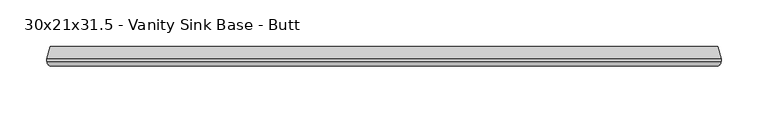
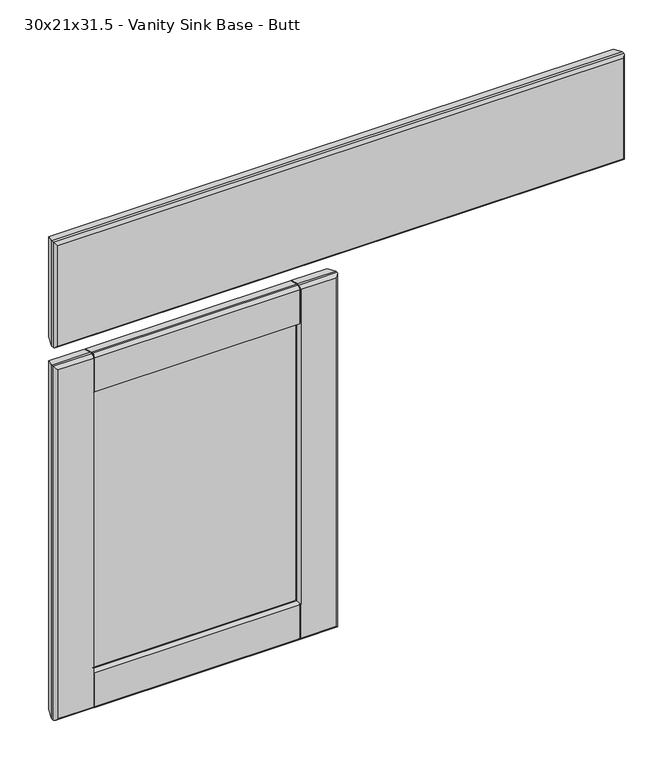
"""IFC4 building model written with IfcOpenShell, lengths in millimetres: furniture geometry, Cabinet-Base-Merillat-Double_Door-Marlin : 30x21x31.5 - Vanity Sink Base - Butt."""

from ifc_helpers import new_model, si_unit, frame, origin, place, context, project, spatial, polyline, circle_curve, ellipse_curve, outline, extrude, source, transform, mapped, element, save
from ifc_brep_helpers import plane_surface, cylinder_surface, advanced_brep


def furniture_30x21x31_5_vanity_sink_base_butt_a027e388(model_context):
    return source(origin(), model_context, "Body", "SolidModel", [
        advanced_brep(
        [(-336.9408026, -629.92, 771.6035075), (-336.9408026, -629.92, 638.0964925), (374.4162124, -629.92, 638.0964925), (374.4162124, -629.92, 771.6035075), (-336.5320951, -609.6, 638.5052), (-336.5320951, -609.6, 771.1948), (374.0075049, -609.6, 771.1948), (374.0075049, -609.6, 638.5052), (-340.0372951, -625.4496, 774.7), (-340.0372951, -622.681, 774.7), (-340.0372951, -622.681, 635.0), (-340.0372951, -625.4496, 635.0), (377.5127049, -622.681, 635.0), (377.5127049, -625.4496, 635.0), (377.5127049, -622.681, 774.7), (377.5127049, -625.4496, 774.7)],
        [
            (0, 1),
            (1, 2),
            (2, 3),
            (3, 0),
            (4, 5),
            (5, 6),
            (6, 7),
            (7, 4),
            (8, 9),
            (9, 10),
            (10, 11),
            (11, 8),
            (10, 12),
            (12, 13),
            (13, 11),
            (12, 14),
            (14, 15),
            (15, 13),
            (8, 15),
            (14, 9),
            (11, 1, ellipse_curve(frame((-335.2620951, -625.4496, 639.7752), z_axis=(-0.7071067811865475, 0.0, 0.7071067811865475), x_axis=(-0.7071067811865474, 0.0, -0.7071067811865476)), 6.7531526, 4.7752)),
            (0, 8, ellipse_curve(frame((-335.2620951, -625.4496, 769.9248), z_axis=(-0.7071067811865475, 0.0, -0.7071067811865475), x_axis=(0.7071067811865474, 0.0, -0.7071067811865476)), 6.7531526, 4.7752)),
            (4, 10),
            (9, 5),
            (13, 2, ellipse_curve(frame((372.7375049, -625.4496, 639.7752), z_axis=(-0.7071067811865475, 0.0, -0.7071067811865475), x_axis=(0.7071067811865476, 0.0, -0.7071067811865474)), 6.7531526, 4.7752)),
            (7, 12),
            (15, 3, ellipse_curve(frame((372.7375049, -625.4496, 769.9248), z_axis=(0.7071067811865475, 0.0, -0.7071067811865475), x_axis=(0.7071067811865474, 0.0, 0.7071067811865476)), 6.7531526, 4.7752)),
            (6, 14),
        ],
        [
            plane_surface(frame((-340.0372951, -629.92, 774.7), z_axis=(0.0, -1.0, 0.0), x_axis=(0.0, 0.0, -1.0))),
            plane_surface(frame((-340.0372951, -609.6, 774.7), z_axis=(0.0, 1.0, 0.0), x_axis=(0.0, 0.0, 1.0))),
            plane_surface(frame((-340.0372951, -629.92, 774.7), z_axis=(-1.0, 0.0, 0.0), x_axis=(0.0, 1.0, 0.0))),
            plane_surface(frame((-340.0372951, -629.92, 635.0), z_axis=(0.0, 0.0, -1.0), x_axis=(0.0, 1.0, 0.0))),
            plane_surface(frame((377.5127049, -629.92, 635.0), z_axis=(1.0, 0.0, 0.0), x_axis=(0.0, 1.0, 0.0))),
            plane_surface(frame((377.5127049, -629.92, 774.7), z_axis=(0.0, 0.0, 1.0), x_axis=(0.0, 1.0, 0.0))),
            cylinder_surface(frame((-335.2620951, -625.4496, 774.7), z_axis=(0.0, 0.0, -1.0), x_axis=(0.0, 1.0, 0.0)), 4.7752),
            plane_surface(frame((-340.0372951, -622.681, 774.7), z_axis=(-0.9659229350723619, 0.25882983502910506, 0.0), x_axis=(0.0, 0.0, -1.0))),
            cylinder_surface(frame((-340.0372951, -625.4496, 639.7752), z_axis=(1.0, 0.0, 0.0), x_axis=(0.0, 1.0, 0.0)), 4.7752),
            plane_surface(frame((-340.0372951, -622.681, 635.0), z_axis=(0.0, 0.25882983502910506, -0.9659229350723619), x_axis=(1.0, 0.0, 0.0))),
            cylinder_surface(frame((372.7375049, -625.4496, 635.0), z_axis=(0.0, 0.0, 1.0), x_axis=(0.0, 1.0, 0.0)), 4.7752),
            plane_surface(frame((377.5127049, -622.681, 635.0), z_axis=(0.9659229350723619, 0.25882983502910506, 0.0), x_axis=(0.0, 0.0, 1.0))),
            cylinder_surface(frame((377.5127049, -625.4496, 769.9248), z_axis=(-1.0, 0.0, 0.0), x_axis=(0.0, 1.0, 0.0)), 4.7752),
            plane_surface(frame((377.5127049, -622.681, 774.7), z_axis=(0.0, 0.25882983502910506, 0.9659229350723619), x_axis=(-1.0, 0.0, 0.0))),
        ],
        [
            (0, [[1, 2, 3, 4]]),
            (1, [[5, 6, 7, 8]]),
            (2, [[9, 10, 11, 12]]),
            (3, [[-11, 13, 14, 15]]),
            (4, [[-14, 16, 17, 18]]),
            (5, [[-9, 19, -17, 20]]),
            (6, [[21, -1, 22, -12]]),
            (7, [[23, -10, 24, -5]]),
            (8, [[-21, -15, 25, -2]]),
            (9, [[-23, -8, 26, -13]]),
            (10, [[-25, -18, 27, -3]]),
            (11, [[-26, -7, 28, -16]]),
            (12, [[-22, -4, -27, -19]]),
            (13, [[-24, -20, -28, -6]]),
        ],
    ),
        advanced_brep(
        [(-340.0372951, -625.4496, 609.6), (-340.0372951, -625.4496, 139.7), (-336.9408026, -629.92, 142.7964925), (-336.9408026, -629.92, 606.5035075), (-340.0372951, -622.681, 609.6), (-340.0372951, -622.681, 139.7), (-336.5320951, -609.6, 606.0948), (-336.5320951, -609.6, 143.2052), (-291.8361323, -609.6, 561.3988372), (-291.4660006, -610.39375, 561.0287055), (-289.3848416, -614.85681, 558.9475465), (-289.3848416, -614.85681, 190.3524535), (-291.4660006, -610.39375, 188.2712945), (-291.8361323, -609.6, 187.9011628), (-290.784611, -617.0969093, 560.347316), (-290.784611, -617.0969093, 188.952684), (-305.1122951, -617.347, 574.675), (-305.1122951, -617.347, 174.625), (-305.1122951, -622.173, 574.675), (-305.1122951, -622.173, 174.625), (-290.784611, -622.4230907, 560.347316), (-290.784611, -622.4230907, 188.952684), (-289.3848416, -624.66319, 558.9475465), (-289.3848416, -624.66319, 190.3524535), (-291.4660006, -629.12625, 561.0287055), (-291.8332649, -629.9138508, 561.3959698), (-291.8361323, -629.92, 187.9011628), (-291.4660006, -629.12625, 188.2712945), (14.0537124, -629.92, 142.7964925), (-31.0140137, -629.92, 142.7964925), (-31.0140137, -625.4496, 139.7), (17.1502049, -625.4496, 139.7), (-291.8332649, -625.4496, 139.7), (-291.8332649, -629.92, 142.7964925), (-290.2457649, -625.4496, 139.7), (-32.6015137, -625.4496, 139.7), (-32.6015137, -629.92, 142.7964925), (-290.2457649, -629.92, 142.7964925), (-31.0140137, -622.681, 139.7), (17.1502049, -622.681, 139.7), (-291.8332649, -622.681, 139.7), (-290.2457649, -622.681, 139.7), (-32.6015137, -622.681, 139.7), (-31.0140137, -609.6, 143.2052), (13.6450049, -609.6, 143.2052), (-290.2457649, -609.6, 143.2052), (-32.6015137, -609.6, 143.2052), (-291.8332649, -609.6, 143.2052), (-33.5022486, -614.85681, 190.3524535), (-31.4210895, -610.39375, 188.2712945), (-32.6015137, -610.39375, 188.2712945), (-32.6015137, -609.6, 187.9011628), (-290.2457649, -609.6, 187.9011628), (-290.2457649, -610.39375, 188.2712945), (-32.1024791, -617.0969093, 188.952684), (-17.7747951, -617.347, 174.625), (-17.7747951, -622.173, 174.625), (-32.1024791, -622.4230907, 188.952684), (-33.5022486, -624.66319, 190.3524535), (-290.2457649, -629.12625, 188.2712945), (-290.2457649, -629.92, 187.9011628), (-32.6015137, -629.92, 187.9011628), (-32.6015137, -629.12625, 188.2712945), (-31.4210895, -629.12625, 188.2712945), (17.1502049, -625.4496, 609.6), (14.0537124, -629.92, 606.5035075), (17.1502049, -622.681, 609.6), (13.6450049, -609.6, 606.0948), (-31.0509578, -609.6, 187.9011628), (-33.5022486, -614.85681, 558.9475465), (-31.4210895, -610.39375, 561.0287055), (-31.0509578, -609.6, 561.3988372), (-32.1024791, -617.0969093, 560.347316), (-17.7747951, -617.347, 574.675), (-17.7747951, -622.173, 574.675), (-32.1024791, -622.4230907, 560.347316), (-33.5022486, -624.66319, 558.9475465), (-31.0509578, -629.92, 187.9011628), (-31.0509578, -629.92, 561.3988372), (-31.4210895, -629.12625, 561.0287055), (-291.8332649, -629.92, 606.5035075), (-291.8332649, -625.4496, 609.6), (-31.0140137, -625.4496, 609.6), (-31.0140137, -629.92, 606.5035075), (-32.6015137, -625.4496, 609.6), (-290.2457649, -625.4496, 609.6), (-290.2457649, -629.92, 606.5035075), (-32.6015137, -629.92, 606.5035075), (-291.8332649, -622.681, 609.6), (-31.0140137, -622.681, 609.6), (-32.6015137, -622.681, 609.6), (-290.2457649, -622.681, 609.6), (-291.8332649, -609.6, 606.0948), (-31.0140137, -609.6, 606.0948), (-32.6015137, -609.6, 606.0948), (-290.2457649, -609.6, 606.0948), (-32.6015137, -609.6, 561.3988372), (-290.2457649, -609.6, 561.3988372), (-290.2457649, -610.39375, 561.0287055), (-32.6015137, -610.39375, 561.0287055), (-32.6015137, -629.12625, 561.0287055), (-32.6015137, -629.92, 561.3988372), (-290.2457649, -629.92, 561.3988372), (-290.2457649, -629.12625, 561.0287055), (-32.6015137, -629.12625, 606.3526052), (-32.6015137, -625.4496, 608.80625), (-32.6015137, -622.7855037, 608.80625), (-32.6015137, -610.39375, 605.4857412), (-31.0140137, -610.39375, 561.0287055), (-31.0140137, -610.39375, 605.4857412), (-31.0140137, -622.7855037, 608.80625), (-31.0140137, -625.4496, 608.80625), (-31.0140137, -629.12625, 606.3526052), (-31.0140137, -629.12625, 561.0287055), (-291.8332649, -629.12625, 561.0287055), (-291.8332649, -629.12625, 606.3526052), (-291.8332649, -625.4496, 608.80625), (-291.8332649, -622.7855037, 608.80625), (-291.8332649, -610.39375, 605.4857412), (-291.8332649, -610.39375, 561.0287055), (-290.2457649, -610.39375, 605.4857412), (-290.2457649, -622.7855037, 608.80625), (-290.2457649, -625.4496, 608.80625), (-290.2457649, -629.12625, 606.3526052), (-291.8332649, -610.39375, 188.2712945), (-291.8332649, -610.39375, 143.8142588), (-291.8332649, -622.7855037, 140.49375), (-291.8332649, -625.4496, 140.49375), (-291.8332649, -629.12625, 142.9473948), (-291.8332649, -629.12625, 188.2712945), (-290.2457649, -629.12625, 142.9473948), (-290.2457649, -625.4496, 140.49375), (-290.2457649, -622.7855037, 140.49375), (-290.2457649, -610.39375, 143.8142588), (-32.6015137, -610.39375, 143.8142588), (-32.6015137, -622.7855037, 140.49375), (-32.6015137, -625.4496, 140.49375), (-32.6015137, -629.12625, 142.9473948), (-31.0140137, -629.12625, 188.2712945), (-31.0140137, -629.12625, 142.9473948), (-31.0140137, -625.4496, 140.49375), (-31.0140137, -622.7855037, 140.49375), (-31.0140137, -610.39375, 143.8142588), (-31.0140137, -610.39375, 188.2712945)],
        [
            (0, 1),
            (1, 2, ellipse_curve(frame((-335.2620951, -625.4496, 144.4752), z_axis=(-0.7071067811865475, 0.0, 0.7071067811865475), x_axis=(0.7071067811865474, 0.0, 0.7071067811865476)), 6.7531526, 4.7752)),
            (2, 3),
            (3, 0, ellipse_curve(frame((-335.2620951, -625.4496, 604.8248), z_axis=(-0.7071067811865475, 0.0, -0.7071067811865475), x_axis=(-0.7071067811865474, 0.0, 0.7071067811865476)), 6.7531526, 4.7752)),
            (0, 4),
            (4, 5),
            (5, 1),
            (4, 6),
            (6, 7),
            (7, 5),
            (8, 9),
            (9, 10),
            (10, 11),
            (11, 12),
            (12, 13),
            (13, 8),
            (10, 14, ellipse_curve(frame((-290.8120951, -615.5223492, 560.3748), z_axis=(-0.7071067811865475, 0.0, -0.7071067811865475), x_axis=(-0.7071067811865474, 0.0, 0.7071067811865476)), 2.2271035, 1.5748)),
            (14, 15),
            (15, 11, ellipse_curve(frame((-290.8120951, -615.5223492, 188.9252), z_axis=(-0.7071067811865475, 0.0, 0.7071067811865475), x_axis=(0.7071067811865474, 0.0, 0.7071067811865476)), 2.2271035, 1.5748)),
            (14, 16),
            (16, 17),
            (17, 15),
            (16, 18),
            (18, 19),
            (19, 17),
            (18, 20),
            (20, 21),
            (21, 19),
            (20, 22, ellipse_curve(frame((-290.8120951, -623.9976508, 560.3748), z_axis=(-0.7071067811865475, 0.0, -0.7071067811865475), x_axis=(-0.7071067811865474, 0.0, 0.7071067811865476)), 2.2271035, 1.5748)),
            (22, 23),
            (23, 21, ellipse_curve(frame((-290.8120951, -623.9976508, 188.9252), z_axis=(-0.7071067811865475, 0.0, 0.7071067811865475), x_axis=(0.7071067811865474, 0.0, 0.7071067811865476)), 2.2271035, 1.5748)),
            (22, 24),
            (24, 25),
            (25, 26),
            (26, 27),
            (27, 23),
            (28, 29),
            (29, 30, circle_curve(frame((-31.0140137, -625.4496, 144.4752), z_axis=(1.0, 0.0, 0.0), x_axis=(0.0, 1.0, 0.0)), 4.7752)),
            (30, 31),
            (31, 28, ellipse_curve(frame((12.3750049, -625.4496, 144.4752), z_axis=(-0.7071067811865475, 0.0, -0.7071067811865475), x_axis=(-0.7071067811865476, 0.0, 0.7071067811865474)), 6.7531526, 4.7752)),
            (1, 32),
            (32, 33, circle_curve(frame((-291.8332649, -625.4496, 144.4752), z_axis=(-1.0, 0.0, 0.0), x_axis=(0.0, 1.0, 0.0)), 4.7752)),
            (33, 2),
            (34, 35),
            (35, 36, circle_curve(frame((-32.6015137, -625.4496, 144.4752), z_axis=(-1.0, 0.0, 0.0), x_axis=(0.0, 1.0, 0.0)), 4.7752)),
            (36, 37),
            (37, 34, circle_curve(frame((-290.2457649, -625.4496, 144.4752), z_axis=(1.0, 0.0, 0.0), x_axis=(0.0, 1.0, 0.0)), 4.7752)),
            (30, 38),
            (38, 39),
            (39, 31),
            (5, 40),
            (40, 32),
            (41, 42),
            (42, 35),
            (34, 41),
            (38, 43),
            (43, 44),
            (44, 39),
            (45, 46),
            (46, 42),
            (41, 45),
            (7, 47),
            (47, 40),
            (48, 49),
            (49, 50),
            (50, 51),
            (51, 52),
            (52, 53),
            (53, 12),
            (11, 48),
            (15, 54),
            (54, 48, ellipse_curve(frame((-32.0749951, -615.5223492, 188.9252), z_axis=(-0.7071067811865475, 0.0, -0.7071067811865475), x_axis=(-0.7071067811865476, 0.0, 0.7071067811865474)), 2.2271035, 1.5748)),
            (17, 55),
            (55, 54),
            (19, 56),
            (56, 55),
            (21, 57),
            (57, 56),
            (23, 58),
            (58, 57, ellipse_curve(frame((-32.0749951, -623.9976508, 188.9252), z_axis=(-0.7071067811865475, 0.0, -0.7071067811865475), x_axis=(-0.7071067811865476, 0.0, 0.7071067811865474)), 2.2271035, 1.5748)),
            (27, 59),
            (59, 60),
            (60, 61),
            (61, 62),
            (62, 63),
            (63, 58),
            (31, 64),
            (64, 65, ellipse_curve(frame((12.3750049, -625.4496, 604.8248), z_axis=(0.7071067811865475, 0.0, -0.7071067811865475), x_axis=(-0.7071067811865474, 0.0, -0.7071067811865476)), 6.7531526, 4.7752)),
            (65, 28),
            (39, 66),
            (66, 64),
            (44, 67),
            (67, 66),
            (68, 49),
            (48, 69),
            (69, 70),
            (70, 71),
            (71, 68),
            (54, 72),
            (72, 69, ellipse_curve(frame((-32.0749951, -615.5223492, 560.3748), z_axis=(0.7071067811865475, 0.0, -0.7071067811865475), x_axis=(-0.7071067811865474, 0.0, -0.7071067811865476)), 2.2271035, 1.5748)),
            (55, 73),
            (73, 72),
            (56, 74),
            (74, 73),
            (57, 75),
            (75, 74),
            (58, 76),
            (76, 75, ellipse_curve(frame((-32.0749951, -623.9976508, 560.3748), z_axis=(0.7071067811865475, 0.0, -0.7071067811865475), x_axis=(-0.7071067811865474, 0.0, -0.7071067811865476)), 2.2271035, 1.5748)),
            (63, 77),
            (77, 78),
            (78, 79),
            (79, 76),
            (3, 80),
            (80, 81, circle_curve(frame((-291.8332649, -625.4496, 604.8248), z_axis=(-1.0, 0.0, 0.0), x_axis=(0.0, 1.0, 0.0)), 4.7752)),
            (81, 0),
            (64, 82),
            (82, 83, circle_curve(frame((-31.0140137, -625.4496, 604.8248), z_axis=(1.0, 0.0, 0.0), x_axis=(0.0, 1.0, 0.0)), 4.7752)),
            (83, 65),
            (84, 85),
            (85, 86, circle_curve(frame((-290.2457649, -625.4496, 604.8248), z_axis=(1.0, 0.0, 0.0), x_axis=(0.0, 1.0, 0.0)), 4.7752)),
            (86, 87),
            (87, 84, circle_curve(frame((-32.6015137, -625.4496, 604.8248), z_axis=(-1.0, 0.0, 0.0), x_axis=(0.0, 1.0, 0.0)), 4.7752)),
            (81, 88),
            (88, 4),
            (66, 89),
            (89, 82),
            (90, 91),
            (91, 85),
            (84, 90),
            (88, 92),
            (92, 6),
            (67, 93),
            (93, 89),
            (94, 95),
            (95, 91),
            (90, 94),
            (51, 46),
            (45, 52),
            (43, 68),
            (71, 93),
            (92, 8),
            (13, 47),
            (96, 97),
            (97, 95),
            (94, 96),
            (9, 98),
            (98, 97),
            (96, 99),
            (99, 70),
            (69, 10),
            (72, 14),
            (73, 16),
            (74, 18),
            (75, 20),
            (76, 22),
            (79, 100),
            (100, 101),
            (101, 102),
            (102, 103),
            (103, 24),
            (33, 26),
            (25, 80),
            (36, 61),
            (60, 37),
            (83, 78),
            (77, 29),
            (86, 102),
            (101, 87),
            (100, 104),
            (104, 105, circle_curve(frame((-32.6015137, -625.4496, 604.8248), z_axis=(-1.0, 0.0, 0.0), x_axis=(0.0, 0.0, 1.0)), 3.98145)),
            (105, 106),
            (106, 107),
            (107, 99),
            (71, 108),
            (108, 109),
            (109, 110),
            (110, 111),
            (111, 112, circle_curve(frame((-31.0140137, -625.4496, 604.8248), z_axis=(1.0, 0.0, 0.0), x_axis=(0.0, 0.0, 1.0)), 3.98145)),
            (112, 113),
            (113, 78),
            (113, 79),
            (112, 104),
            (111, 105),
            (110, 106),
            (109, 107),
            (108, 70),
            (25, 114),
            (114, 115),
            (115, 116, circle_curve(frame((-291.8332649, -625.4496, 604.8248), z_axis=(-1.0, 0.0, 0.0), x_axis=(0.0, 0.0, 1.0)), 3.98145)),
            (116, 117),
            (117, 118),
            (118, 119),
            (119, 8),
            (98, 120),
            (120, 121),
            (121, 122),
            (122, 123, circle_curve(frame((-290.2457649, -625.4496, 604.8248), z_axis=(1.0, 0.0, 0.0), x_axis=(0.0, 0.0, 1.0)), 3.98145)),
            (123, 103),
            (24, 114),
            (123, 115),
            (122, 116),
            (121, 117),
            (120, 118),
            (9, 119),
            (13, 124),
            (124, 125),
            (125, 126),
            (126, 127),
            (127, 128, circle_curve(frame((-291.8332649, -625.4496, 144.4752), z_axis=(-1.0, 0.0, 0.0), x_axis=(0.0, 0.0, 1.0)), 3.98145)),
            (128, 129),
            (129, 26),
            (59, 130),
            (130, 131, circle_curve(frame((-290.2457649, -625.4496, 144.4752), z_axis=(1.0, 0.0, 0.0), x_axis=(0.0, 0.0, 1.0)), 3.98145)),
            (131, 132),
            (132, 133),
            (133, 53),
            (12, 124),
            (133, 125),
            (132, 126),
            (131, 127),
            (130, 128),
            (27, 129),
            (50, 134),
            (134, 135),
            (135, 136),
            (136, 137, circle_curve(frame((-32.6015137, -625.4496, 144.4752), z_axis=(-1.0, 0.0, 0.0), x_axis=(0.0, 0.0, 1.0)), 3.98145)),
            (137, 62),
            (138, 139),
            (139, 140, circle_curve(frame((-31.0140137, -625.4496, 144.4752), z_axis=(1.0, 0.0, 0.0), x_axis=(0.0, 0.0, 1.0)), 3.98145)),
            (140, 141),
            (141, 142),
            (142, 143),
            (143, 68),
            (77, 138),
            (63, 138),
            (143, 49),
            (142, 134),
            (141, 135),
            (140, 136),
            (139, 137),
        ],
        [
            cylinder_surface(frame((-335.2620951, -625.4496, 609.6), z_axis=(0.0, 0.0, 1.0), x_axis=(0.0, 1.0, 0.0)), 4.7752),
            plane_surface(frame((-340.0372951, -625.4496, 609.6), z_axis=(-1.0, 0.0, 0.0), x_axis=(0.0, 0.0, -1.0))),
            plane_surface(frame((-340.0372951, -622.681, 609.6), z_axis=(-0.9659229350723619, 0.25882983502910506, 0.0), x_axis=(0.0, 0.0, -1.0))),
            plane_surface(frame((-291.8361323, -609.6, 561.3988372), z_axis=(0.9063077870366099, 0.4226182617407856, 0.0), x_axis=(0.0, 0.0, -1.0))),
            cylinder_surface(frame((-290.8120951, -615.5223492, 609.6), z_axis=(0.0, 0.0, 1.0000000000000002), x_axis=(0.01745240643729364, -0.9998476951563912, 0.0)), 1.5748),
            plane_surface(frame((-290.784611, -617.0969093, 560.347316), z_axis=(0.017452406437322144, -0.9998476951563906, 0.0), x_axis=(0.0, 0.0, -1.0))),
            plane_surface(frame((-305.1122951, -617.347, 574.675), z_axis=(1.0, 0.0, 0.0), x_axis=(0.0, 0.0, -1.0))),
            plane_surface(frame((-305.1122951, -622.173, 574.675), z_axis=(0.01745240643727848, 0.9998476951563914, 0.0), x_axis=(0.0, 0.0, -1.0))),
            cylinder_surface(frame((-290.8120951, -623.9976508, 609.6), z_axis=(0.0, 0.0, 1.0000000000000002), x_axis=(0.9063077870367326, -0.42261826174052236, 0.0)), 1.5748),
            plane_surface(frame((-289.3848416, -624.66319, 558.9475465), z_axis=(0.9063077870366333, -0.4226182617407352, 0.0), x_axis=(0.0, 0.0, -1.0))),
            cylinder_surface(frame((-340.0372951, -625.4496, 144.4752), z_axis=(-1.0, 0.0, 0.0), x_axis=(0.0, 1.0, 0.0)), 4.7752),
            plane_surface(frame((-340.0372951, -625.4496, 139.7), z_axis=(0.0, 0.0, -1.0), x_axis=(1.0, 0.0, 0.0))),
            plane_surface(frame((-340.0372951, -622.681, 139.7), z_axis=(0.0, 0.25882983502910506, -0.9659229350723619), x_axis=(1.0, 0.0, 0.0))),
            plane_surface(frame((-291.8361323, -609.6, 187.9011628), z_axis=(0.0, 0.4226182617407856, 0.9063077870366099), x_axis=(1.0, 0.0, 0.0))),
            cylinder_surface(frame((-340.0372951, -615.5223492, 188.9252), z_axis=(-1.0000000000000002, 0.0, 0.0), x_axis=(0.0, -0.9998476951563912, 0.01745240643729364)), 1.5748),
            plane_surface(frame((-290.784611, -617.0969093, 188.952684), z_axis=(0.0, -0.9998476951563906, 0.017452406437322144), x_axis=(1.0, 0.0, 0.0))),
            plane_surface(frame((-305.1122951, -617.347, 174.625), z_axis=(0.0, 0.0, 1.0), x_axis=(1.0, 0.0, 0.0))),
            plane_surface(frame((-305.1122951, -622.173, 174.625), z_axis=(0.0, 0.9998476951563914, 0.01745240643727848), x_axis=(1.0, 0.0, 0.0))),
            cylinder_surface(frame((-340.0372951, -623.9976508, 188.9252), z_axis=(-1.0000000000000002, 0.0, 0.0), x_axis=(0.0, -0.42261826174052236, 0.9063077870367326)), 1.5748),
            plane_surface(frame((-289.3848416, -624.66319, 190.3524535), z_axis=(0.0, -0.4226182617407352, 0.9063077870366333), x_axis=(1.0, 0.0, 0.0))),
            cylinder_surface(frame((12.3750049, -625.4496, 139.7), z_axis=(0.0, 0.0, -1.0), x_axis=(0.0, 1.0, 0.0)), 4.7752),
            plane_surface(frame((17.1502049, -625.4496, 139.7), z_axis=(1.0, 0.0, 0.0), x_axis=(0.0, 0.0, 1.0))),
            plane_surface(frame((17.1502049, -622.681, 139.7), z_axis=(0.9659229350723619, 0.25882983502910506, 0.0), x_axis=(0.0, 0.0, 1.0))),
            plane_surface(frame((-31.0509578, -609.6, 187.9011628), z_axis=(-0.9063077870366099, 0.4226182617407856, 0.0), x_axis=(0.0, 0.0, 1.0))),
            cylinder_surface(frame((-32.0749951, -615.5223492, 139.7), z_axis=(0.0, 0.0, -1.0000000000000002), x_axis=(-0.01745240643729364, -0.9998476951563912, 0.0)), 1.5748),
            plane_surface(frame((-32.1024791, -617.0969093, 188.952684), z_axis=(-0.017452406437322144, -0.9998476951563906, 0.0), x_axis=(0.0, 0.0, 1.0))),
            plane_surface(frame((-17.7747951, -617.347, 174.625), z_axis=(-1.0, 0.0, 0.0), x_axis=(0.0, 0.0, 1.0))),
            plane_surface(frame((-17.7747951, -622.173, 174.625), z_axis=(-0.01745240643727848, 0.9998476951563914, 0.0), x_axis=(0.0, 0.0, 1.0))),
            cylinder_surface(frame((-32.0749951, -623.9976508, 139.7), z_axis=(0.0, 0.0, -1.0000000000000002), x_axis=(-0.9063077870367326, -0.42261826174052236, 0.0)), 1.5748),
            plane_surface(frame((-33.5022486, -624.66319, 190.3524535), z_axis=(-0.9063077870366333, -0.4226182617407352, 0.0), x_axis=(0.0, 0.0, 1.0))),
            cylinder_surface(frame((17.1502049, -625.4496, 604.8248), z_axis=(1.0, 0.0, 0.0), x_axis=(0.0, 1.0, 0.0)), 4.7752),
            plane_surface(frame((17.1502049, -625.4496, 609.6), z_axis=(0.0, 0.0, 1.0), x_axis=(-1.0, 0.0, 0.0))),
            plane_surface(frame((17.1502049, -622.681, 609.6), z_axis=(0.0, 0.25882983502910506, 0.9659229350723619), x_axis=(-1.0, 0.0, 0.0))),
            plane_surface(frame((13.6450049, -609.6, 606.0948), z_axis=(0.0, 1.0, 0.0), x_axis=(-1.0, 0.0, 0.0))),
            plane_surface(frame((-31.0509578, -609.6, 561.3988372), z_axis=(0.0, 0.4226182617407856, -0.9063077870366099), x_axis=(-1.0, 0.0, 0.0))),
            cylinder_surface(frame((17.1502049, -615.5223492, 560.3748), z_axis=(1.0000000000000002, 0.0, 0.0), x_axis=(0.0, -0.9998476951563912, -0.01745240643729364)), 1.5748),
            plane_surface(frame((-32.1024791, -617.0969093, 560.347316), z_axis=(0.0, -0.9998476951563906, -0.017452406437322144), x_axis=(-1.0, 0.0, 0.0))),
            plane_surface(frame((-17.7747951, -617.347, 574.675), z_axis=(0.0, 0.0, -1.0), x_axis=(-1.0, 0.0, 0.0))),
            plane_surface(frame((-17.7747951, -622.173, 574.675), z_axis=(0.0, 0.9998476951563914, -0.01745240643727848), x_axis=(-1.0, 0.0, 0.0))),
            cylinder_surface(frame((17.1502049, -623.9976508, 560.3748), z_axis=(1.0000000000000002, 0.0, 0.0), x_axis=(0.0, -0.42261826174052236, -0.9063077870367326)), 1.5748),
            plane_surface(frame((-33.5022486, -624.66319, 558.9475465), z_axis=(0.0, -0.4226182617407352, -0.9063077870366333), x_axis=(-1.0, 0.0, 0.0))),
            plane_surface(frame((-31.0509578, -629.92, 561.3988372), z_axis=(0.0, -1.0, 0.0), x_axis=(-1.0, 0.0, 0.0))),
            plane_surface(frame((-32.6015137, -629.92, 561.3988372), z_axis=(1.0, 0.0, 0.0), x_axis=(0.0, 0.9063077870366297, -0.42261826174074285))),
            plane_surface(frame((-31.0140137, -629.92, 561.3988372), z_axis=(-1.0, 0.0, 0.0), x_axis=(0.0, -0.9063077870366297, 0.42261826174074285))),
            plane_surface(frame((-32.6015137, -629.92, 561.3988372), z_axis=(0.0, 0.42261826174074285, 0.9063077870366297), x_axis=(1.0, 0.0, 0.0))),
            plane_surface(frame((-32.6015137, -629.12625, 561.0287055), z_axis=(0.0, -1.0, 0.0), x_axis=(1.0, 0.0, 0.0))),
            cylinder_surface(frame((-31.0140137, -625.4496, 604.8248), z_axis=(1.0, 0.0, 0.0), x_axis=(0.0, 0.0, 1.0)), 3.98145),
            plane_surface(frame((-32.6015137, -625.4496, 608.80625), z_axis=(0.0, 0.0, 1.0), x_axis=(1.0, 0.0, 0.0))),
            plane_surface(frame((-32.6015137, -622.7855037, 608.80625), z_axis=(0.0, 0.25882983502916584, 0.9659229350723456), x_axis=(1.0, 0.0, 0.0))),
            plane_surface(frame((-32.6015137, -610.39375, 605.4857412), z_axis=(0.0, 1.0, 0.0), x_axis=(1.0, 0.0, 0.0))),
            plane_surface(frame((-32.6015137, -610.39375, 561.0287055), z_axis=(0.0, -0.42261826174077916, 0.9063077870366127), x_axis=(1.0, 0.0, 0.0))),
            plane_surface(frame((-291.8332649, -629.92, 561.3988372), z_axis=(1.0, 0.0, 0.0), x_axis=(0.0, 0.9063077870366253, -0.4226182617407524))),
            plane_surface(frame((-290.2457649, -629.92, 561.3988372), z_axis=(-1.0, 0.0, 0.0), x_axis=(0.0, -0.9063077870366253, 0.4226182617407524))),
            plane_surface(frame((-291.8332649, -629.92, 561.3988372), z_axis=(0.0, 0.4226182617407524, 0.9063077870366253), x_axis=(1.0, 0.0, 0.0))),
            plane_surface(frame((-291.8332649, -629.12625, 561.0287055), z_axis=(0.0, -1.0, 0.0), x_axis=(1.0, 0.0, 0.0))),
            cylinder_surface(frame((-290.2457649, -625.4496, 604.8248), z_axis=(1.0, 0.0, 0.0), x_axis=(0.0, 0.0, 1.0)), 3.98145),
            plane_surface(frame((-291.8332649, -625.4496, 608.80625), z_axis=(0.0, 0.0, 1.0), x_axis=(1.0, 0.0, 0.0))),
            plane_surface(frame((-291.8332649, -622.7855037, 608.80625), z_axis=(0.0, 0.25882983502916573, 0.9659229350723457), x_axis=(1.0, 0.0, 0.0))),
            plane_surface(frame((-291.8332649, -610.39375, 605.4857412), z_axis=(0.0, 1.0, 0.0), x_axis=(1.0, 0.0, 0.0))),
            plane_surface(frame((-291.8332649, -610.39375, 561.0287055), z_axis=(0.0, -0.4226182617407701, 0.906307787036617), x_axis=(1.0, 0.0, 0.0))),
            plane_surface(frame((-291.8332649, -625.4496, 149.2504), z_axis=(1.0, 0.0, 0.0), x_axis=(0.0, -1.0, 0.0))),
            plane_surface(frame((-290.2457649, -625.4496, 149.2504), z_axis=(-1.0, 0.0, 0.0), x_axis=(0.0, 1.0, 0.0))),
            plane_surface(frame((-291.8332649, -609.6, 187.9011628), z_axis=(0.0, -0.4226182617407918, -0.906307787036607), x_axis=(1.0, 0.0, 0.0))),
            plane_surface(frame((-291.8332649, -610.39375, 188.2712945), z_axis=(0.0, 1.0, 0.0), x_axis=(1.0, 0.0, 0.0))),
            plane_surface(frame((-291.8332649, -610.39375, 143.8142588), z_axis=(0.0, 0.25882983502943896, -0.9659229350722724), x_axis=(1.0, 0.0, 0.0))),
            plane_surface(frame((-291.8332649, -622.7855037, 140.49375), z_axis=(0.0, 0.0, -1.0), x_axis=(1.0, 0.0, 0.0))),
            cylinder_surface(frame((-290.2457649, -625.4496, 144.4752), z_axis=(1.0, 0.0, 0.0), x_axis=(0.0, 0.0, 1.0)), 3.98145),
            plane_surface(frame((-291.8332649, -629.12625, 142.9473948), z_axis=(0.0, -1.0, 0.0), x_axis=(1.0, 0.0, 0.0))),
            plane_surface(frame((-291.8332649, -629.12625, 188.2712945), z_axis=(0.0, 0.42261826174073464, -0.9063077870366336), x_axis=(1.0, 0.0, 0.0))),
            plane_surface(frame((-32.6015137, -629.12625, 188.2712945), z_axis=(1.0, 0.0, 0.0), x_axis=(0.0, -0.9063077870366323, -0.4226182617407374))),
            plane_surface(frame((-31.0140137, -629.12625, 188.2712945), z_axis=(-1.0, 0.0, 0.0), x_axis=(0.0, 0.9063077870366323, 0.4226182617407374))),
            plane_surface(frame((-32.6015137, -629.12625, 188.2712945), z_axis=(0.0, 0.4226182617407374, -0.9063077870366323), x_axis=(1.0, 0.0, 0.0))),
            plane_surface(frame((-32.6015137, -609.6, 187.9011628), z_axis=(0.0, -0.42261826174081374, -0.9063077870365968), x_axis=(1.0, 0.0, 0.0))),
            plane_surface(frame((-32.6015137, -610.39375, 188.2712945), z_axis=(0.0, 1.0, 0.0), x_axis=(1.0, 0.0, 0.0))),
            plane_surface(frame((-32.6015137, -610.39375, 143.8142588), z_axis=(0.0, 0.25882983502943885, -0.9659229350722726), x_axis=(1.0, 0.0, 0.0))),
            plane_surface(frame((-32.6015137, -622.7855037, 140.49375), z_axis=(0.0, 0.0, -1.0), x_axis=(1.0, 0.0, 0.0))),
            cylinder_surface(frame((-31.0140137, -625.4496, 144.4752), z_axis=(1.0, 0.0, 0.0), x_axis=(0.0, 0.0, 1.0)), 3.98145),
            plane_surface(frame((-32.6015137, -629.12625, 142.9473948), z_axis=(0.0, -1.0, 0.0), x_axis=(1.0, 0.0, 0.0))),
        ],
        [
            (0, [[1, 2, 3, 4]]),
            (1, [[5, 6, 7, -1]]),
            (2, [[8, 9, 10, -6]]),
            (3, [[11, 12, 13, 14, 15, 16]]),
            (4, [[17, 18, 19, -13]]),
            (5, [[20, 21, 22, -18]]),
            (6, [[23, 24, 25, -21]]),
            (7, [[26, 27, 28, -24]]),
            (8, [[29, 30, 31, -27]]),
            (9, [[32, 33, 34, 35, 36, -30]]),
            (10, [[37, 38, 39, 40]]),
            (10, [[41, 42, 43, -2]]),
            (10, [[44, 45, 46, 47]]),
            (11, [[-39, 48, 49, 50]]),
            (11, [[51, 52, -41, -7]]),
            (11, [[53, 54, -44, 55]]),
            (12, [[-49, 56, 57, 58]]),
            (12, [[59, 60, -53, 61]]),
            (12, [[62, 63, -51, -10]]),
            (13, [[64, 65, 66, 67, 68, 69, -14, 70]]),
            (14, [[71, 72, -70, -19]]),
            (15, [[73, 74, -71, -22]]),
            (16, [[75, 76, -73, -25]]),
            (17, [[77, 78, -75, -28]]),
            (18, [[79, 80, -77, -31]]),
            (19, [[-36, 81, 82, 83, 84, 85, 86, -79]]),
            (20, [[87, 88, 89, -40]]),
            (21, [[90, 91, -87, -50]]),
            (22, [[92, 93, -90, -58]]),
            (23, [[94, -64, 95, 96, 97, 98]]),
            (24, [[99, 100, -95, -72]]),
            (25, [[101, 102, -99, -74]]),
            (26, [[103, 104, -101, -76]]),
            (27, [[105, 106, -103, -78]]),
            (28, [[107, 108, -105, -80]]),
            (29, [[-86, 109, 110, 111, 112, -107]]),
            (30, [[113, 114, 115, -4]]),
            (30, [[116, 117, 118, -88]]),
            (30, [[119, 120, 121, 122]]),
            (31, [[-115, 123, 124, -5]]),
            (31, [[125, 126, -116, -91]]),
            (31, [[127, 128, -119, 129]]),
            (32, [[-124, 130, 131, -8]]),
            (32, [[132, 133, -125, -93]]),
            (32, [[134, 135, -127, 136]]),
            (33, [[-67, 137, -59, 138]]),
            (33, [[-57, 139, -98, 140, -132, -92]]),
            (33, [[-131, 141, -16, 142, -62, -9]]),
            (33, [[143, 144, -134, 145]]),
            (34, [[-12, 146, 147, -143, 148, 149, -96, 150]]),
            (35, [[-150, -100, 151, -17]]),
            (36, [[-151, -102, 152, -20]]),
            (37, [[-152, -104, 153, -23]]),
            (38, [[-153, -106, 154, -26]]),
            (39, [[-154, -108, 155, -29]]),
            (40, [[-112, 156, 157, 158, 159, 160, -32, -155]]),
            (41, [[-43, 161, -34, 162, -113, -3]]),
            (41, [[-46, 163, -83, 164]]),
            (41, [[-118, 165, -110, 166, -37, -89]]),
            (41, [[-121, 167, -158, 168]]),
            (42, [[-148, -145, -136, -129, -122, -168, -157, 169, 170, 171, 172, 173]]),
            (43, [[-165, -117, -126, -133, -140, 174, 175, 176, 177, 178, 179, 180]]),
            (44, [[181, -111, -180]]),
            (45, [[-156, -181, -179, 182, -169]]),
            (46, [[-182, -178, 183, -170]]),
            (47, [[-183, -177, 184, -171]]),
            (48, [[-184, -176, 185, -172]]),
            (49, [[-185, -175, 186, -149, -173]]),
            (50, [[-97, -186, -174]]),
            (51, [[-141, -130, -123, -114, -162, 187, 188, 189, 190, 191, 192, 193]]),
            (52, [[-159, -167, -120, -128, -135, -144, -147, 194, 195, 196, 197, 198]]),
            (53, [[-33, 199, -187]]),
            (54, [[-199, -160, -198, 200, -188]]),
            (55, [[-200, -197, 201, -189]]),
            (56, [[-201, -196, 202, -190]]),
            (57, [[-202, -195, 203, -191]]),
            (58, [[-203, -194, -146, 204, -192]]),
            (59, [[-204, -11, -193]]),
            (60, [[-161, -42, -52, -63, -142, 205, 206, 207, 208, 209, 210, 211]]),
            (61, [[-68, -138, -61, -55, -47, -164, -82, 212, 213, 214, 215, 216]]),
            (62, [[-15, 217, -205]]),
            (63, [[-217, -69, -216, 218, -206]]),
            (64, [[-218, -215, 219, -207]]),
            (65, [[-219, -214, 220, -208]]),
            (66, [[-220, -213, 221, -209]]),
            (67, [[-221, -212, -81, 222, -210]]),
            (68, [[-222, -35, -211]]),
            (69, [[-84, -163, -45, -54, -60, -137, -66, 223, 224, 225, 226, 227]]),
            (70, [[228, 229, 230, 231, 232, 233, -139, -56, -48, -38, -166, 234]]),
            (71, [[-109, 235, -234]]),
            (72, [[236, -94, -233]]),
            (73, [[-65, -236, -232, 237, -223]]),
            (74, [[-237, -231, 238, -224]]),
            (75, [[-238, -230, 239, -225]]),
            (76, [[-239, -229, 240, -226]]),
            (77, [[-240, -228, -235, -85, -227]]),
        ],
    ),
        extrude(outline(polyline([(-17.7747951, -622.173), (-305.1122951, -622.173), (-305.1122951, -617.347), (-17.7747951, -617.347), (-17.7747951, -622.173)])), frame((0.0, 0.0, 174.625), z_axis=(0.0, 0.0, 1.0), x_axis=(1.0, 0.0, 0.0)), (0.0, 0.0, 1.0), 400.05),
    ])


if __name__ == "__main__":
    model = new_model("IFC4")
    model_context = context("Model", 3, world=origin())
    ifc_project = project(units=[si_unit("LENGTHUNIT", "METRE", prefix="MILLI")], contexts=[model_context])
    site = spatial("IfcSite", under=ifc_project)
    building = spatial("IfcBuilding", under=site)
    placement = place(None, origin())
    furniture_30x21x31_5_vanity_sink_base_butt_shape = furniture_30x21x31_5_vanity_sink_base_butt_a027e388(model_context)
    element("IfcFurniture", 1, ObjectType="Cabinet-Base-Merillat-Double_Door-Marlin : 30x21x31.5 - Vanity Sink Base - Butt", at=placement, inside=building, context=model_context, shape_type="MappedRepresentation", body=[
        mapped(furniture_30x21x31_5_vanity_sink_base_butt_shape, transform((0.0, 0.0, 0.0), x_axis=(1.0, 0.0, 0.0), y_axis=(0.0, 1.0, 0.0), z_axis=(0.0, 0.0, 1.0))),
    ])
    save(model, "model.ifc")

# Revit data of these elements
# Type "Cabinet-Base-Merillat-Double_Door-Marlin : 30x21x31.5 - Vanity Sink Base - Butt"
#   URL = "http://www.merillat.com"
#   Toe Kick Note = "Toe Kick Covering is not included. To be purchased Separately."
#   Product Line = "Express"
#   Product Page URL = "http://www.merillat.com//our-products/rooms/bathroom"
#   Product Group = "Vanity Cabinet"
#   Product Documentation Link = "http://merillatbusiness.com/customer-resources/product-line-resources/merillat-classic/"
#   Model = "VSB30B"
#   Manufacturer = "Merillat"
#   Finish = "Wood"
#   Description = "Vanity Sink Base Butt Door"
#   Construction Type = "Deep Sink Base"
#   Cabinet Construction Note = "No shelf, cabinets w/ a \"B\" suffix have BUTT doors without a center frame stile,  VSB39, VSB42. VSB3935 and VSB4235 have a double door with a frame center stile, All cabinets have one full-width drawer front except VSB42 and VSB4235 which have two drawer fronts"
#   Assembly Code = "C1030410"
#   Toe Kick Height = 0' - 4 1/2"
#   Toe Kick Depth = 0' - 2 25/32"
#   Top and Bottom Spacing = 0' - 1"
#   Side Spacing = 0' - 0 7/8"
#   Cabinet Shell = 0' - 0 3/8"
#   Door Spacing = 0' - 0 1/8"
#   Depth = 1' - 9"
#   Height = 2' - 7 1/2"
#   Width = 2' - 6"
#   Cabinet Drawer Width = 2' - 4 1/4"
#   Cabinet Drawer Height = 0' - 5 1/2"
#   Cabinet Drawer 2 Drawer Width = 1' - 2 1/16"
#   Cabinet Door Width = 1' - 2 1/16"
#   Cabinet Door Height = 1' - 6 1/2"
#   COBie.Type = no
#   Two Drawer = no
#   Elevation Swing Line = yes
#   Partial Overlay = yes
#   One Drawer = yes
#   Full Overlay = no
#   Butt Option = yes
#   Toe Kick Material = Wood - Merillat - Raw Particle Board
#   Door Drawer Material = Wood - Merillat - Pecan(1)
#   Cabinet Material = Wood - Merillat - Pecan(1)
#   Cabinet Drawer Style 2 Drawer = element 819256
#   Cabinet Drawer Style = element 819255
#   Cabinet Door Style = element 819254
# Element 1 (IfcFurniture, "Cabinet-Base-Merillat-Double_Door-Marlin : 30x21x31.5 - Vanity Sink Base - Butt")
#   Materials on its faces: "Wood - Merillat - Pecan(1)", "Wood - Merillat - Raw Particle Board"
# Materials
#   "Wood - Merillat - Raw Particle Board": class "Plastic", colour RGB 80 80 80, transparency 0, Description = "Plastic Laminate - Navy", Cost = 0
#   "Wood - Merillat - Pecan(1)": class "Wood", colour RGB 108 67 43, transparency 0, Cost = 0
